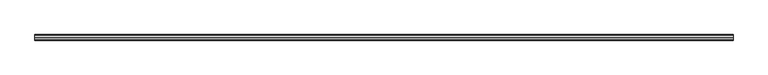
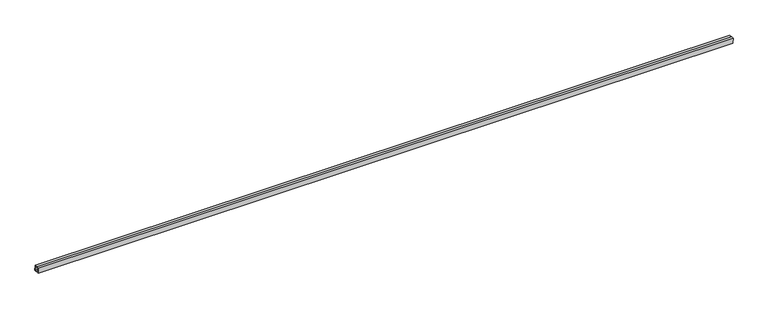
"""IFC4 building model written with IfcOpenShell, lengths in millimetres: proxy geometry, Inner panel:Inner panel:1:Inner panel:1 : Inner panel:Inner panel:300324:2:Inner panel:1:Inner panel:1 : Inner panel:Inner panel:300324:2 : Inner panel:Inner panel:1:Inner panel:1 : Inner panel:Inner panel:300324:300043:53 : Inner panel:Inner panel:1:Inner panel:1 : Inner panel:Inner panel:300324:2:Inner panel:1:Inner panel:1 : Inner panel:Inner panel:300324:2 : Inner panel:Inner panel:1:Inner panel:1 : Inner panel:Inner panel:300324:300043:308120."""

from ifc_helpers import new_model, si_unit, frame, origin, place, context, project, spatial, polyline, outline, extrude, source, transform, mapped, element, save


def generic_models_0b58f102(model_context):
    return source(origin(), model_context, "Body", "SweptSolid", [
        extrude(outline(polyline([(-580481.3921913, 3888.2024845), (-580463.1517681, 3888.9625021), (-580461.5656444, 3850.895532), (-580499.6326145, 3849.3094083), (-580501.2187382, 3887.3763783), (-580482.9783151, 3888.136396), (-580482.8791823, 3885.7572103), (-580498.7404199, 3885.0963254), (-580497.3525616, 3851.7877266), (-580464.0439628, 3853.1755849), (-580465.431821, 3886.4841837), (-580481.2930586, 3885.8232988), (-580481.3921913, 3888.2024845)])), frame((659327.2367238, 0.0, 0.0), z_axis=(1.0, 0.0, 0.0), x_axis=(0.0, 1.0, 0.0)), (0.0, 0.0, 1.0), 4876.8),
    ])


if __name__ == "__main__":
    model = new_model("IFC4")
    model_context = context("Model", 3, world=origin())
    ifc_project = project(units=[si_unit("LENGTHUNIT", "METRE", prefix="MILLI")], contexts=[model_context])
    site = spatial("IfcSite", under=ifc_project)
    building = spatial("IfcBuilding", under=site)
    placement = place(None, origin())
    generic_models_shape = generic_models_0b58f102(model_context)
    element("IfcBuildingElementProxy", 1, Name="Inner panel:Inner panel:1:Inner panel:1 : Inner panel:Inner panel:300324:2:Inner panel:1:Inner panel:1 : Inner panel:Inner panel:300324:2 : Inner panel:Inner panel:1:Inner panel:1 : Inner panel:Inner panel:300324:300043:53 : Inner panel:Inner panel:1:Inner panel:1 : Inner panel:Inner panel:300324:2:Inner panel:1:Inner panel:1 : Inner panel:Inner panel:300324:2 : Inner panel:Inner panel:1:Inner panel:1 : Inner panel:Inner panel:300324:300043:308120", ObjectType="Inner panel:Inner panel:1:Inner panel:1 : Inner panel:Inner panel:300324:2:Inner panel:1:Inner panel:1 : Inner panel:Inner panel:300324:2 : Inner panel:Inner panel:1:Inner panel:1 : Inner panel:Inner panel:300324:300043:53 : Inner panel:Inner panel:1:Inner panel:1 : Inner panel:Inner panel:300324:2:Inner panel:1:Inner panel:1 : Inner panel:Inner panel:300324:2 : Inner panel:Inner panel:1:Inner panel:1 : Inner panel:Inner panel:300324:300043:308120", at=placement, inside=building, context=model_context, shape_type="MappedRepresentation", body=[
        mapped(generic_models_shape, transform((0.0, 0.0, 0.0), x_axis=(1.0, 0.0, 0.0), y_axis=(0.0, 1.0, 0.0), z_axis=(0.0, 0.0, 1.0))),
    ])
    save(model, "model.ifc")

# Revit data of these elements
# Type "Inner panel:Inner panel:1:Inner panel:1 : Inner panel:Inner panel:300324:2:Inner panel:1:Inner panel:1 : Inner panel:Inner panel:300324:2 : Inner panel:Inner panel:1:Inner panel:1 : Inner panel:Inner panel:300324:300043:53 : Inner panel:Inner panel:1:Inner panel:1 : Inner panel:Inner panel:300324:2:Inner panel:1:Inner panel:1 : Inner panel:Inner panel:300324:2 : Inner panel:Inner panel:1:Inner panel:1 : Inner panel:Inner panel:300324:300043:308120"
#   NameOverride = "Inner panel:Inner panel:1:Inner panel:1 : Inner panel:Inner panel:300324:2:Inner panel:1:Inner panel:1 : Inner panel:Inner panel:300324:2 : Inner panel:Inner panel:1:Inner panel:1 : Inner panel:Inner panel:300324:300043:308120"
#   ObjectTypeOverride = "Inner panel:1:Inner panel:1 : Inner panel:Inner panel:300324:2 : Inner panel:Inner panel:1:Inner panel:1 : Inner panel:Inner panel:300324:300043"
#   Reference = "Inner panel"
#   Tag = "308120"
# Element 1 (IfcBuildingElementProxy, "Inner panel:Inner panel:1:Inner panel:1 : Inner panel:Inner panel:300324:2:Inner panel:1:Inner panel:1 : Inner panel:Inner panel:300324:2 : Inner panel:Inner panel:1:Inner panel:1 : Inner panel:Inner panel:300324:300043:53 : Inner panel:Inner panel:1:Inner panel:1 : Inner panel:Inner panel:300324:2:Inner panel:1:Inner panel:1 : Inner panel:Inner panel:300324:2 : Inner panel:Inner panel:1:Inner panel:1 : Inner panel:Inner panel:300324:300043:308120")
#   Materials on its faces: "1 1/2\" X 1 1/2\" SPLIT-SEAM SQUARE TUBING (~24\" CANTILEVER FROM C.L. OF GLULAM)"
# Materials
#   "1 1/2\" X 1 1/2\" SPLIT-SEAM SQUARE TUBING (~24\" CANTILEVER FROM C.L. OF GLULAM)": class "Unassigned", colour RGB 202 201 200, transparency 0, Cost = 0
